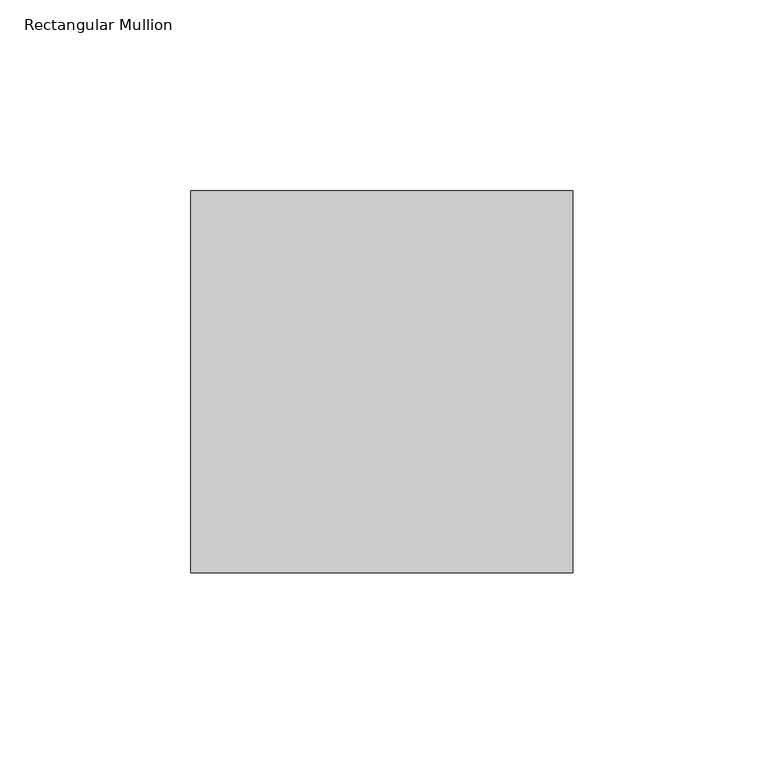
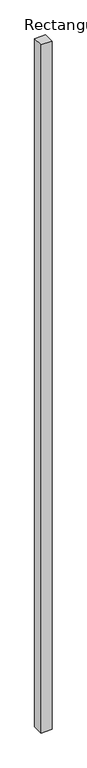
"""IFC4 building model written with IfcOpenShell, lengths in millimetres: member geometry, Rectangular Mullion : 알루미늄_Rectangular Cap_100 x100."""

from ifc_helpers import new_model, si_unit, frame, origin, place, context, project, spatial, polyline, outline, extrude, source, transform, mapped, element, save


def rectangular_mullion_46d195e2(model_context):
    return source(origin(), model_context, "Body", "SweptSolid", [
        extrude(outline(polyline([(0.0, 50.0), (0.0, -50.0), (-100.0, -50.0), (-100.0, 50.0), (0.0, 50.0)])), frame((0.0, 0.0, -6569.0), z_axis=(0.0, 0.0, 1.0), x_axis=(1.0, 0.0, 0.0)), (0.0, 0.0, 1.0), 6569.0),
    ])


if __name__ == "__main__":
    model = new_model("IFC4")
    model_context = context("Model", 3, world=origin())
    ifc_project = project(units=[si_unit("LENGTHUNIT", "METRE", prefix="MILLI")], contexts=[model_context])
    site = spatial("IfcSite", under=ifc_project)
    building = spatial("IfcBuilding", under=site)
    placement = place(None, origin())
    rectangular_mullion_shape = rectangular_mullion_46d195e2(model_context)
    element("IfcMember", 1, ObjectType="Rectangular Mullion : 알루미늄_Rectangular Cap_100 x100", at=placement, inside=building, context=model_context, shape_type="MappedRepresentation", body=[
        mapped(rectangular_mullion_shape, transform((0.0, 0.0, 0.0), x_axis=(1.0, 0.0, 0.0), y_axis=(0.0, 1.0, 0.0), z_axis=(0.0, 0.0, 1.0))),
    ])
    save(model, "model.ifc")

# Revit data of these elements
# Type "Rectangular Mullion : 알루미늄_Rectangular Cap_100 x100"
#   built-in parameter 1007304 = 0.328084 (stored number, unit not read)
#   built-in parameter 1007301 = 0.164042 (stored number, unit not read)
#   built-in parameter 1007300 = 0.164042 (stored number, unit not read)
# Element 1 (IfcMember, "Rectangular Mullion : 알루미늄_Rectangular Cap_100 x100")
#   Materials on its faces: "00_Metal_Stainless Steel"
# Materials
#   "00_Metal_Stainless Steel": class "Metal", colour RGB 148 148 148, transparency 0, Description = "Steel", Cost = 0
